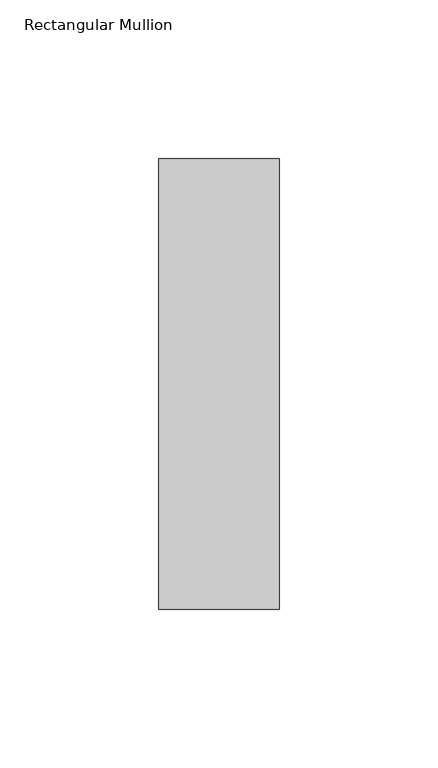
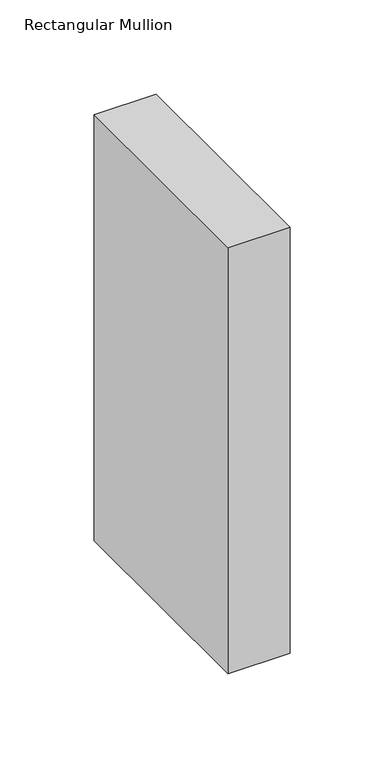
"""IFC4 building model written with IfcOpenShell, lengths in millimetres: member geometry, Rectangular Mullion : NLRS_21_CWM_hsb-regel 38x142_gen_rsf."""

import ifcopenshell
import ifcopenshell.guid

model = None  # the IFC model being written
_history = None  # IfcOwnerHistory: only IFC2X3 demands one
_inside = {}  # id of a spatial element -> (the spatial element, [elements in it])
_under = {}  # id of a project, library or spatial element -> (it, [spatial elements below it])
_declared = {}  # id of a project -> (the project, [libraries it declares])
_typed = {}  # id of a type object -> (the type object, [elements of that type])
_made_of = {}  # id of a material, layer set ... -> (it, [elements and type objects made of it])


def new_model(schema):
    """Start an empty IFC model of exactly this schema.

    Asked for "IFC4X3", IfcOpenShell would pick the latest addendum, in which some entities
    have other attributes; the version numbers below select the first issue.
    IFC2X3 requires an IfcOwnerHistory on every rooted entity: one is made here for all.
    """
    global model, _history
    if schema == "IFC4X3":
        model = ifcopenshell.file(schema_version=(4, 3, 0, 0))
    else:
        model = ifcopenshell.file(schema=schema)
    _inside.clear()
    _under.clear()
    _declared.clear()
    _typed.clear()
    _made_of.clear()
    _history = None
    if model.schema == "IFC2X3":
        org = make("IfcOrganization", Name="unknown")
        user = make(
            "IfcPersonAndOrganization",
            ThePerson=make("IfcPerson", FamilyName="unknown"),
            TheOrganization=org,
        )
        app = make(
            "IfcApplication",
            ApplicationDeveloper=org,
            Version="unknown",
            ApplicationFullName="unknown",
            ApplicationIdentifier="unknown",
        )
        _history = make(
            "IfcOwnerHistory",
            OwningUser=user,
            OwningApplication=app,
            ChangeAction="ADDED",
            CreationDate=0,
        )
    return model


def make(cls, **values):
    """One entity of the class cls with the attributes given. An attribute that is None is left unset."""
    return model.create_entity(
        cls, **{name: value for name, value in values.items() if value is not None}
    )


def rooted(cls, **values):
    """An entity with a GlobalId (a new one), such as an element, a storey or a relation."""
    return make(cls, GlobalId=ifcopenshell.guid.new(), OwnerHistory=_history, **values)


def si_unit(unit_type, name, prefix=None):
    """IfcSIUnit, for example si_unit("LENGTHUNIT", "METRE", prefix="MILLI")."""
    return make("IfcSIUnit", UnitType=unit_type, Prefix=prefix, Name=name)


def assignment(units):
    """IfcUnitAssignment: the units of a project."""
    return None if units is None else make("IfcUnitAssignment", Units=units)


def point(xyz):
    """IfcCartesianPoint."""
    return None if xyz is None else make("IfcCartesianPoint", Coordinates=xyz)


def direction(xyz):
    """IfcDirection."""
    return None if xyz is None else make("IfcDirection", DirectionRatios=xyz)


def frame(location, z_axis=None, x_axis=None):
    """IfcAxis2Placement3D, a coordinate frame: its origin and axes. An axis left out is left unset."""
    return make(
        "IfcAxis2Placement3D",
        Location=point(location),
        Axis=direction(z_axis),
        RefDirection=direction(x_axis),
    )


def origin():
    """The frame at (0, 0, 0) with its axes left unset."""
    return frame((0.0, 0.0, 0.0))


def place(relative_to, where):
    """IfcLocalPlacement: puts the frame where relative to a parent placement (None: the world)."""
    return make(
        "IfcLocalPlacement", PlacementRelTo=relative_to, RelativePlacement=where
    )


def context(
    kind, dimensions, precision=None, world=None, true_north=None, identifier=None
):
    """IfcGeometricRepresentationContext, for example the 3D "Model" context."""
    return make(
        "IfcGeometricRepresentationContext",
        ContextIdentifier=identifier,
        ContextType=kind,
        CoordinateSpaceDimension=dimensions,
        Precision=precision,
        WorldCoordinateSystem=world,
        TrueNorth=true_north,
    )


def project(units=None, contexts=None):
    """IfcProject with its units and contexts."""
    return rooted(
        "IfcProject",
        Name="project",
        RepresentationContexts=contexts,
        UnitsInContext=assignment(units),
    )


def spatial(cls, under=None, at=None, **own):
    """A site, building, storey or space (cls), placed at a placement, below another one or the project."""
    s = rooted(cls, ObjectPlacement=at, **own)
    if under is not None:
        _under.setdefault(under.id(), (under, []))[1].append(s)
    return s


def polyline(points):
    """IfcPolyline through the points."""
    return make("IfcPolyline", Points=[point(p) for p in points])


def outline(outer, holes=None, kind="AREA"):
    """IfcArbitraryClosedProfileDef: a profile drawn as a closed curve; with holes, ...WithVoids."""
    if holes is None:
        return make("IfcArbitraryClosedProfileDef", ProfileType=kind, OuterCurve=outer)
    return make(
        "IfcArbitraryProfileDefWithVoids",
        ProfileType=kind,
        OuterCurve=outer,
        InnerCurves=holes,
    )


def extrude(swept, where, along, depth):
    """IfcExtrudedAreaSolid: the profile swept, set in the frame where, extruded along a direction by depth."""
    return make(
        "IfcExtrudedAreaSolid",
        SweptArea=swept,
        Position=where,
        ExtrudedDirection=direction(along),
        Depth=depth,
    )


def shape(context_of_items, identifier, shape_type, items):
    """IfcShapeRepresentation: the items that make up one representation, for example the "Body"."""
    return make(
        "IfcShapeRepresentation",
        ContextOfItems=context_of_items,
        RepresentationIdentifier=identifier,
        RepresentationType=shape_type,
        Items=items,
    )


def source(mapping_origin, context_of_items, identifier, shape_type, items):
    """IfcRepresentationMap: a shape defined once, which mapped items show again and again."""
    return make(
        "IfcRepresentationMap",
        MappingOrigin=mapping_origin,
        MappedRepresentation=shape(context_of_items, identifier, shape_type, items),
    )


def transform(
    local_origin,
    x_axis=None,
    y_axis=None,
    z_axis=None,
    scale=None,
    scale2=None,
    scale3=None,
    uniform=True,
):
    """IfcCartesianTransformationOperator3D, or its non-uniform kind. x_axis, y_axis, z_axis: its Axis1, 2, 3."""
    if uniform:
        return make(
            "IfcCartesianTransformationOperator3D",
            Axis1=direction(x_axis),
            Axis2=direction(y_axis),
            LocalOrigin=point(local_origin),
            Scale=scale,
            Axis3=direction(z_axis),
        )
    return make(
        "IfcCartesianTransformationOperator3DnonUniform",
        Axis1=direction(x_axis),
        Axis2=direction(y_axis),
        LocalOrigin=point(local_origin),
        Scale=scale,
        Axis3=direction(z_axis),
        Scale2=scale2,
        Scale3=scale3,
    )


def mapped(mapping_source, mapping_target):
    """IfcMappedItem: shows the shape of a source again, moved by a transform."""
    return make(
        "IfcMappedItem", MappingSource=mapping_source, MappingTarget=mapping_target
    )


def made_of(thing, what):
    """Note that an element or type object is made of a material, layer set ...; save() writes the relation."""
    if what is not None:
        _made_of.setdefault(what.id(), (what, []))[1].append(thing)
    return thing


def element(
    cls,
    number,
    at=None,
    inside=None,
    cuts=None,
    type_object=None,
    material=None,
    context=None,
    identifier="Body",
    shape_type=None,
    held_by="IfcProductDefinitionShape",
    body=None,
    shapes=None,
    **own,
):
    """One element of the class cls, such as IfcWall. Its Tag is "e" and its number.

    at: its placement. inside: the storey or other place that contains it. cuts: it is an
    opening in that element (IfcRelVoidsElement). A single representation is given by context,
    identifier, shape_type and body (its items); several are given by shapes. held_by: the class
    of the entity that holds the representations. save() writes the other relations.
    """
    e = rooted(cls, Tag="e%d" % number, ObjectPlacement=at, **own)
    if body is not None:
        shapes = [shape(context, identifier, shape_type, body)]
    if shapes is not None:
        e.Representation = make(held_by, Representations=shapes)
    if inside is not None:
        _inside.setdefault(inside.id(), (inside, []))[1].append(e)
    if cuts is not None:
        rooted(
            "IfcRelVoidsElement", RelatingBuildingElement=cuts, RelatedOpeningElement=e
        )
    if type_object is not None:
        _typed.setdefault(type_object.id(), (type_object, []))[1].append(e)
    return made_of(e, material)


def aggregate(whole, parts):
    """IfcRelAggregates: a whole, such as a stair, and the parts it consists of."""
    return rooted("IfcRelAggregates", RelatingObject=whole, RelatedObjects=parts)


def save(model, path):
    """Write the relations noted so far, then the file.

    IfcRelAggregates (storeys below a building ...), IfcRelContainedInSpatialStructure (elements
    in a storey), IfcRelDefinesByType, IfcRelAssociatesMaterial and IfcRelDeclares: one each for
    every whole, place, type object, material and project.
    """
    for whole, parts in _under.values():
        aggregate(whole, parts)
    for where, things in _inside.values():
        rooted(
            "IfcRelContainedInSpatialStructure",
            RelatedElements=things,
            RelatingStructure=where,
        )
    for kind, things in _typed.values():
        rooted("IfcRelDefinesByType", RelatedObjects=things, RelatingType=kind)
    for what, things in _made_of.values():
        rooted("IfcRelAssociatesMaterial", RelatedObjects=things, RelatingMaterial=what)
    for by, libraries in _declared.values():
        rooted("IfcRelDeclares", RelatingContext=by, RelatedDefinitions=libraries)
    model.write(path)


def rectangular_mullion_f581aa4a(model_context):
    return source(origin(), model_context, "Body", "SweptSolid", [
        extrude(outline(polyline([(19.0, -71.0), (-19.0, -71.0), (-19.0, 71.0), (19.0, 71.0), (19.0, -71.0)])), frame((0.0, 0.0, -276.0), z_axis=(0.0, 0.0, 1.0), x_axis=(1.0, 0.0, 0.0)), (0.0, 0.0, 1.0), 276.0),
    ])


if __name__ == "__main__":
    model = new_model("IFC4")
    model_context = context("Model", 3, world=origin())
    ifc_project = project(units=[si_unit("LENGTHUNIT", "METRE", prefix="MILLI")], contexts=[model_context])
    site = spatial("IfcSite", under=ifc_project)
    building = spatial("IfcBuilding", under=site)
    placement = place(None, origin())
    rectangular_mullion_shape = rectangular_mullion_f581aa4a(model_context)
    element("IfcMember", 1, ObjectType="Rectangular Mullion : NLRS_21_CWM_hsb-regel 38x142_gen_rsf", at=placement, inside=building, context=model_context, shape_type="MappedRepresentation", body=[
        mapped(rectangular_mullion_shape, transform((0.0, 0.0, 0.0), x_axis=(1.0, 0.0, 0.0), y_axis=(0.0, 1.0, 0.0), z_axis=(0.0, 0.0, 1.0))),
    ])
    save(model, "model.ifc")

# Revit data of these elements
# Type "Rectangular Mullion : NLRS_21_CWM_hsb-regel 38x142_gen_rsf"
#   Export Type to IFC As = "IfcWall"
#   Type IfcGUID = "07M7mRoiH1CR8m_RSKIwpF"
#   Assembly Code = "21.10"
#   built-in parameter 1007322 = 0.465879 (stored number, unit not read)
#   built-in parameter 1007321 = 0.062336 (stored number, unit not read)
#   built-in parameter 1007320 = 0.062336 (stored number, unit not read)
# Element 1 (IfcMember, "Rectangular Mullion : NLRS_21_CWM_hsb-regel 38x142_gen_rsf")
#   Materials on its faces: "NLRS_i2_hout naaldhout vuren_gen_rsf"
# Materials
#   "NLRS_i2_hout naaldhout vuren_gen_rsf": class "I - Hout", colour RGB 234 199 147, transparency 0, Keynote = "i2", Manufacturer = "Revit Standards Foundation", URL = "www.revitstandards.org", Description = "hout vuren", Cost = 0
